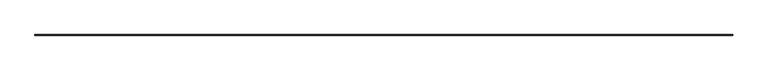
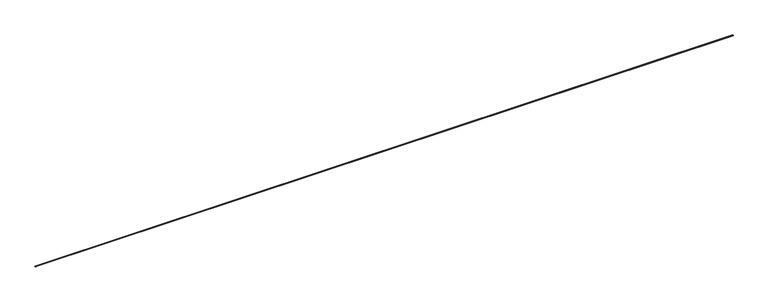
"""IFC4 building model written with IfcOpenShell, lengths in millimetres: proxy geometry, Inner panel:Inner panel:1:Inner panel:1 : Inner panel:Inner panel:300324:2:Inner panel:1:Inner panel:1 : Inner panel:Inner panel:300324:2 : Inner panel:Inner panel:1:Inner panel:1 : Inner panel:Inner panel:300324:300043:49 : Inner panel:Inner panel:1:Inner panel:1 : Inner panel:Inner panel:300324:2:Inner panel:1:Inner panel:1 : Inner panel:Inner panel:300324:2 : Inner panel:Inner panel:1:Inner panel:1 : Inner panel:Inner panel:300324:300043:308120."""

from ifc_helpers import new_model, si_unit, frame, origin, place, context, project, spatial, polyline, outline, extrude, source, transform, mapped, element, save


def generic_models_fb304f62(model_context):
    return source(origin(), model_context, "Body", "SweptSolid", [
        extrude(outline(polyline([(-566869.9020895, 8820.4270332), (-566871.4221248, 8856.9078795), (-566914.300281, 8855.1212897), (-566912.7802458, 8818.6404433), (-566929.4546528, 8817.9456764), (-566929.6118933, 8821.7194493), (-566928.0230159, 8821.7194493), (-566927.9346175, 8819.5978886), (-566914.432458, 8820.1604786), (-566915.9524933, 8856.6413249), (-566869.9020895, 8858.5600917), (-566868.3820542, 8822.0792454), (-566854.8798948, 8822.6418354), (-566854.9710468, 8824.8294845), (-566853.3821694, 8824.8294845), (-566853.2276825, 8821.1218001), (-566869.9020895, 8820.4270332)])), frame((579104.5117239, 0.0, 0.0), z_axis=(1.0, 0.0, 0.0), x_axis=(0.0, 1.0, 0.0)), (0.0, 0.0, 1.0), 88442.8),
    ])


if __name__ == "__main__":
    model = new_model("IFC4")
    model_context = context("Model", 3, world=origin())
    ifc_project = project(units=[si_unit("LENGTHUNIT", "METRE", prefix="MILLI")], contexts=[model_context])
    site = spatial("IfcSite", under=ifc_project)
    building = spatial("IfcBuilding", under=site)
    placement = place(None, origin())
    generic_models_shape = generic_models_fb304f62(model_context)
    element("IfcBuildingElementProxy", 1, Name="Inner panel:Inner panel:1:Inner panel:1 : Inner panel:Inner panel:300324:2:Inner panel:1:Inner panel:1 : Inner panel:Inner panel:300324:2 : Inner panel:Inner panel:1:Inner panel:1 : Inner panel:Inner panel:300324:300043:49 : Inner panel:Inner panel:1:Inner panel:1 : Inner panel:Inner panel:300324:2:Inner panel:1:Inner panel:1 : Inner panel:Inner panel:300324:2 : Inner panel:Inner panel:1:Inner panel:1 : Inner panel:Inner panel:300324:300043:308120", ObjectType="Inner panel:Inner panel:1:Inner panel:1 : Inner panel:Inner panel:300324:2:Inner panel:1:Inner panel:1 : Inner panel:Inner panel:300324:2 : Inner panel:Inner panel:1:Inner panel:1 : Inner panel:Inner panel:300324:300043:49 : Inner panel:Inner panel:1:Inner panel:1 : Inner panel:Inner panel:300324:2:Inner panel:1:Inner panel:1 : Inner panel:Inner panel:300324:2 : Inner panel:Inner panel:1:Inner panel:1 : Inner panel:Inner panel:300324:300043:308120", at=placement, inside=building, context=model_context, shape_type="MappedRepresentation", body=[
        mapped(generic_models_shape, transform((0.0, 0.0, 0.0), x_axis=(1.0, 0.0, 0.0), y_axis=(0.0, 1.0, 0.0), z_axis=(0.0, 0.0, 1.0))),
    ])
    save(model, "model.ifc")

# Revit data of these elements
# Type "Inner panel:Inner panel:1:Inner panel:1 : Inner panel:Inner panel:300324:2:Inner panel:1:Inner panel:1 : Inner panel:Inner panel:300324:2 : Inner panel:Inner panel:1:Inner panel:1 : Inner panel:Inner panel:300324:300043:49 : Inner panel:Inner panel:1:Inner panel:1 : Inner panel:Inner panel:300324:2:Inner panel:1:Inner panel:1 : Inner panel:Inner panel:300324:2 : Inner panel:Inner panel:1:Inner panel:1 : Inner panel:Inner panel:300324:300043:308120"
#   NameOverride = "Inner panel:Inner panel:1:Inner panel:1 : Inner panel:Inner panel:300324:2:Inner panel:1:Inner panel:1 : Inner panel:Inner panel:300324:2 : Inner panel:Inner panel:1:Inner panel:1 : Inner panel:Inner panel:300324:300043:308120"
#   ObjectTypeOverride = "Inner panel:1:Inner panel:1 : Inner panel:Inner panel:300324:2 : Inner panel:Inner panel:1:Inner panel:1 : Inner panel:Inner panel:300324:300043"
#   Reference = "Inner panel"
#   Tag = "308120"
# Element 1 (IfcBuildingElementProxy, "Inner panel:Inner panel:1:Inner panel:1 : Inner panel:Inner panel:300324:2:Inner panel:1:Inner panel:1 : Inner panel:Inner panel:300324:2 : Inner panel:Inner panel:1:Inner panel:1 : Inner panel:Inner panel:300324:300043:49 : Inner panel:Inner panel:1:Inner panel:1 : Inner panel:Inner panel:300324:2:Inner panel:1:Inner panel:1 : Inner panel:Inner panel:300324:2 : Inner panel:Inner panel:1:Inner panel:1 : Inner panel:Inner panel:300324:300043:308120")
#   Materials on its faces: "1 1/2\" HAT CHANNELS - SEE STRUCT. DWGs"
# Materials
#   "1 1/2\" HAT CHANNELS - SEE STRUCT. DWGs": class "Metal", colour RGB 189 187 185, transparency 0, Description = "Structural steel 50ksi", Cost = 0
